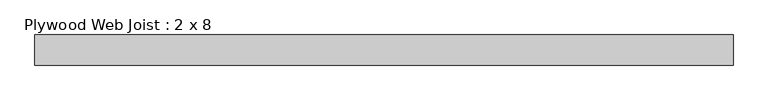
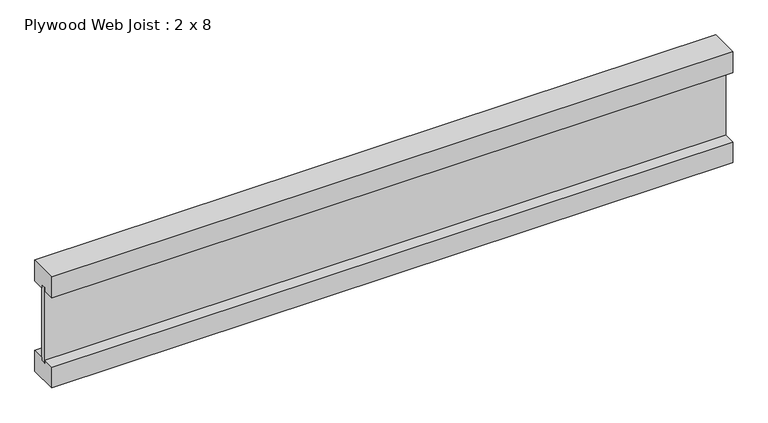
"""IFC4 building model written with IfcOpenShell, lengths in millimetres: beam geometry, Plywood Web Joist : 2 x 8."""

from ifc_helpers import new_model, si_unit, frame, origin, place, context, project, spatial, polyline, outline, extrude, source, transform, mapped, element, save


def plywood_web_joist_2_x_8_69fe57bf(model_context):
    return source(origin(), model_context, "Body", "SweptSolid", [
        extrude(outline(polyline([(-25.4, 101.6), (25.4, 101.6), (25.4, 63.5), (4.7625, 63.5), (4.7625, 69.85), (-4.7625, 69.85), (-4.7625, 63.5), (-25.4, 63.5), (-25.4, 101.6)])), frame((-589.0383025, 0.0, 0.0), z_axis=(1.0, 0.0, 0.0), x_axis=(0.0, 1.0, 0.0)), (0.0, 0.0, 1.0), 1178.0766049),
        extrude(outline(polyline([(25.4, -63.5), (25.4, -101.6), (-25.4, -101.6), (-25.4, -63.5), (-4.7625, -63.5), (-4.7625, -69.1160374), (4.7625, -69.1160374), (4.7625, -63.5), (25.4, -63.5)])), frame((-589.0383025, 0.0, 0.0), z_axis=(1.0, 0.0, 0.0), x_axis=(0.0, 1.0, 0.0)), (0.0, 0.0, 1.0), 1178.0766049),
        extrude(outline(polyline([(589.0383025, 4.7625), (589.0383025, -4.7625), (-589.0383025, -4.7625), (-589.0383025, 4.7625), (589.0383025, 4.7625)])), frame((0.0, 0.0, -69.1160374), z_axis=(0.0, 0.0, 1.0), x_axis=(1.0, 0.0, 0.0)), (0.0, 0.0, 1.0), 138.9660374),
    ])


if __name__ == "__main__":
    model = new_model("IFC4")
    model_context = context("Model", 3, world=origin())
    ifc_project = project(units=[si_unit("LENGTHUNIT", "METRE", prefix="MILLI")], contexts=[model_context])
    site = spatial("IfcSite", under=ifc_project)
    building = spatial("IfcBuilding", under=site)
    placement = place(None, origin())
    plywood_web_joist_2_x_8_shape = plywood_web_joist_2_x_8_69fe57bf(model_context)
    element("IfcBeam", 1, ObjectType="Plywood Web Joist : 2 x 8", at=placement, inside=building, context=model_context, shape_type="MappedRepresentation", body=[
        mapped(plywood_web_joist_2_x_8_shape, transform((0.0, 0.0, 0.0), x_axis=(1.0, 0.0, 0.0), y_axis=(0.0, 1.0, 0.0), z_axis=(0.0, 0.0, 1.0))),
    ])
    save(model, "model.ifc")

# Revit data of these elements
# Type "Plywood Web Joist : 2 x 8"
#   Assembly Code = "B10"
#   Length [instance default] = 5' - 0"
#   b = 0' - 2"
#   d = 0' - 8"
#   Structural Material [instance default] = Softwood, Lumber
# Element 1 (IfcBeam, "Plywood Web Joist : 2 x 8")
#   Materials on its faces: "Softwood, Lumber"
# Materials
#   "Softwood, Lumber": class "Wood", colour RGB 144 113 62, transparency 0, Description = "Pinus Echinata", Cost = 0
